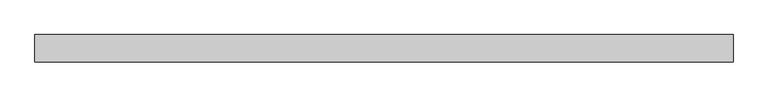
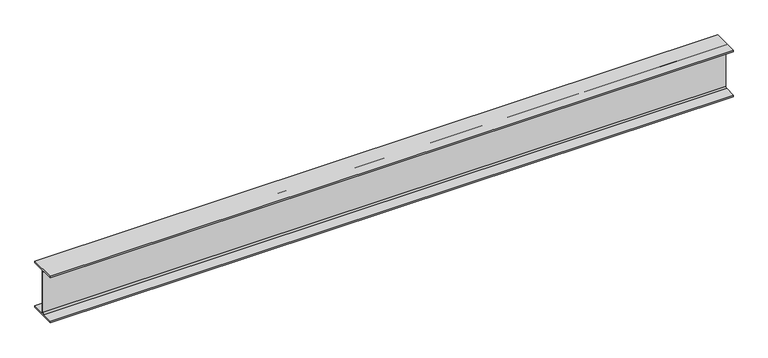
"""IFC4 building model written with IfcOpenShell, lengths in millimetres: beam geometry, Old_Steel Beam_H-KSD3502 : H_SB_ASB_H-482×300x11x15."""

import ifcopenshell
import ifcopenshell.guid

model = None  # the IFC model being written
_history = None  # IfcOwnerHistory: only IFC2X3 demands one
_inside = {}  # id of a spatial element -> (the spatial element, [elements in it])
_under = {}  # id of a project, library or spatial element -> (it, [spatial elements below it])
_declared = {}  # id of a project -> (the project, [libraries it declares])
_typed = {}  # id of a type object -> (the type object, [elements of that type])
_made_of = {}  # id of a material, layer set ... -> (it, [elements and type objects made of it])


def new_model(schema):
    """Start an empty IFC model of exactly this schema.

    Asked for "IFC4X3", IfcOpenShell would pick the latest addendum, in which some entities
    have other attributes; the version numbers below select the first issue.
    IFC2X3 requires an IfcOwnerHistory on every rooted entity: one is made here for all.
    """
    global model, _history
    if schema == "IFC4X3":
        model = ifcopenshell.file(schema_version=(4, 3, 0, 0))
    else:
        model = ifcopenshell.file(schema=schema)
    _inside.clear()
    _under.clear()
    _declared.clear()
    _typed.clear()
    _made_of.clear()
    _history = None
    if model.schema == "IFC2X3":
        org = make("IfcOrganization", Name="unknown")
        user = make(
            "IfcPersonAndOrganization",
            ThePerson=make("IfcPerson", FamilyName="unknown"),
            TheOrganization=org,
        )
        app = make(
            "IfcApplication",
            ApplicationDeveloper=org,
            Version="unknown",
            ApplicationFullName="unknown",
            ApplicationIdentifier="unknown",
        )
        _history = make(
            "IfcOwnerHistory",
            OwningUser=user,
            OwningApplication=app,
            ChangeAction="ADDED",
            CreationDate=0,
        )
    return model


def make(cls, **values):
    """One entity of the class cls with the attributes given. An attribute that is None is left unset."""
    return model.create_entity(
        cls, **{name: value for name, value in values.items() if value is not None}
    )


def rooted(cls, **values):
    """An entity with a GlobalId (a new one), such as an element, a storey or a relation."""
    return make(cls, GlobalId=ifcopenshell.guid.new(), OwnerHistory=_history, **values)


def si_unit(unit_type, name, prefix=None):
    """IfcSIUnit, for example si_unit("LENGTHUNIT", "METRE", prefix="MILLI")."""
    return make("IfcSIUnit", UnitType=unit_type, Prefix=prefix, Name=name)


def assignment(units):
    """IfcUnitAssignment: the units of a project."""
    return None if units is None else make("IfcUnitAssignment", Units=units)


def point(xyz):
    """IfcCartesianPoint."""
    return None if xyz is None else make("IfcCartesianPoint", Coordinates=xyz)


def direction(xyz):
    """IfcDirection."""
    return None if xyz is None else make("IfcDirection", DirectionRatios=xyz)


def frame(location, z_axis=None, x_axis=None):
    """IfcAxis2Placement3D, a coordinate frame: its origin and axes. An axis left out is left unset."""
    return make(
        "IfcAxis2Placement3D",
        Location=point(location),
        Axis=direction(z_axis),
        RefDirection=direction(x_axis),
    )


def frame_2d(location, x_axis=None):
    """IfcAxis2Placement2D, a coordinate frame in the plane: its origin and x axis."""
    return make(
        "IfcAxis2Placement2D", Location=point(location), RefDirection=direction(x_axis)
    )


def origin():
    """The frame at (0, 0, 0) with its axes left unset."""
    return frame((0.0, 0.0, 0.0))


def place(relative_to, where):
    """IfcLocalPlacement: puts the frame where relative to a parent placement (None: the world)."""
    return make(
        "IfcLocalPlacement", PlacementRelTo=relative_to, RelativePlacement=where
    )


def context(
    kind, dimensions, precision=None, world=None, true_north=None, identifier=None
):
    """IfcGeometricRepresentationContext, for example the 3D "Model" context."""
    return make(
        "IfcGeometricRepresentationContext",
        ContextIdentifier=identifier,
        ContextType=kind,
        CoordinateSpaceDimension=dimensions,
        Precision=precision,
        WorldCoordinateSystem=world,
        TrueNorth=true_north,
    )


def project(units=None, contexts=None):
    """IfcProject with its units and contexts."""
    return rooted(
        "IfcProject",
        Name="project",
        RepresentationContexts=contexts,
        UnitsInContext=assignment(units),
    )


def spatial(cls, under=None, at=None, **own):
    """A site, building, storey or space (cls), placed at a placement, below another one or the project."""
    s = rooted(cls, ObjectPlacement=at, **own)
    if under is not None:
        _under.setdefault(under.id(), (under, []))[1].append(s)
    return s


def polyline(points):
    """IfcPolyline through the points."""
    return make("IfcPolyline", Points=[point(p) for p in points])


def circle_curve(where, radius):
    """IfcCircle in the frame where."""
    return make("IfcCircle", Position=where, Radius=radius)


def trimmed(basis, trim1, trim2, sense, master):
    """IfcTrimmedCurve: the piece of a basis curve between two trims."""
    return make(
        "IfcTrimmedCurve",
        BasisCurve=basis,
        Trim1=trim1,
        Trim2=trim2,
        SenseAgreement=sense,
        MasterRepresentation=master,
    )


def segment(curve, same_sense, transition):
    """IfcCompositeCurveSegment."""
    return make(
        "IfcCompositeCurveSegment",
        Transition=transition,
        SameSense=same_sense,
        ParentCurve=curve,
    )


def composite_curve(segments, self_intersect=None):
    """IfcCompositeCurve: segments joined end to end."""
    return make("IfcCompositeCurve", Segments=segments, SelfIntersect=self_intersect)


def outline(outer, holes=None, kind="AREA"):
    """IfcArbitraryClosedProfileDef: a profile drawn as a closed curve; with holes, ...WithVoids."""
    if holes is None:
        return make("IfcArbitraryClosedProfileDef", ProfileType=kind, OuterCurve=outer)
    return make(
        "IfcArbitraryProfileDefWithVoids",
        ProfileType=kind,
        OuterCurve=outer,
        InnerCurves=holes,
    )


def extrude(swept, where, along, depth):
    """IfcExtrudedAreaSolid: the profile swept, set in the frame where, extruded along a direction by depth."""
    return make(
        "IfcExtrudedAreaSolid",
        SweptArea=swept,
        Position=where,
        ExtrudedDirection=direction(along),
        Depth=depth,
    )


def shape(context_of_items, identifier, shape_type, items):
    """IfcShapeRepresentation: the items that make up one representation, for example the "Body"."""
    return make(
        "IfcShapeRepresentation",
        ContextOfItems=context_of_items,
        RepresentationIdentifier=identifier,
        RepresentationType=shape_type,
        Items=items,
    )


def source(mapping_origin, context_of_items, identifier, shape_type, items):
    """IfcRepresentationMap: a shape defined once, which mapped items show again and again."""
    return make(
        "IfcRepresentationMap",
        MappingOrigin=mapping_origin,
        MappedRepresentation=shape(context_of_items, identifier, shape_type, items),
    )


def transform(
    local_origin,
    x_axis=None,
    y_axis=None,
    z_axis=None,
    scale=None,
    scale2=None,
    scale3=None,
    uniform=True,
):
    """IfcCartesianTransformationOperator3D, or its non-uniform kind. x_axis, y_axis, z_axis: its Axis1, 2, 3."""
    if uniform:
        return make(
            "IfcCartesianTransformationOperator3D",
            Axis1=direction(x_axis),
            Axis2=direction(y_axis),
            LocalOrigin=point(local_origin),
            Scale=scale,
            Axis3=direction(z_axis),
        )
    return make(
        "IfcCartesianTransformationOperator3DnonUniform",
        Axis1=direction(x_axis),
        Axis2=direction(y_axis),
        LocalOrigin=point(local_origin),
        Scale=scale,
        Axis3=direction(z_axis),
        Scale2=scale2,
        Scale3=scale3,
    )


def mapped(mapping_source, mapping_target):
    """IfcMappedItem: shows the shape of a source again, moved by a transform."""
    return make(
        "IfcMappedItem", MappingSource=mapping_source, MappingTarget=mapping_target
    )


def made_of(thing, what):
    """Note that an element or type object is made of a material, layer set ...; save() writes the relation."""
    if what is not None:
        _made_of.setdefault(what.id(), (what, []))[1].append(thing)
    return thing


def element(
    cls,
    number,
    at=None,
    inside=None,
    cuts=None,
    type_object=None,
    material=None,
    context=None,
    identifier="Body",
    shape_type=None,
    held_by="IfcProductDefinitionShape",
    body=None,
    shapes=None,
    **own,
):
    """One element of the class cls, such as IfcWall. Its Tag is "e" and its number.

    at: its placement. inside: the storey or other place that contains it. cuts: it is an
    opening in that element (IfcRelVoidsElement). A single representation is given by context,
    identifier, shape_type and body (its items); several are given by shapes. held_by: the class
    of the entity that holds the representations. save() writes the other relations.
    """
    e = rooted(cls, Tag="e%d" % number, ObjectPlacement=at, **own)
    if body is not None:
        shapes = [shape(context, identifier, shape_type, body)]
    if shapes is not None:
        e.Representation = make(held_by, Representations=shapes)
    if inside is not None:
        _inside.setdefault(inside.id(), (inside, []))[1].append(e)
    if cuts is not None:
        rooted(
            "IfcRelVoidsElement", RelatingBuildingElement=cuts, RelatedOpeningElement=e
        )
    if type_object is not None:
        _typed.setdefault(type_object.id(), (type_object, []))[1].append(e)
    return made_of(e, material)


def aggregate(whole, parts):
    """IfcRelAggregates: a whole, such as a stair, and the parts it consists of."""
    return rooted("IfcRelAggregates", RelatingObject=whole, RelatedObjects=parts)


def save(model, path):
    """Write the relations noted so far, then the file.

    IfcRelAggregates (storeys below a building ...), IfcRelContainedInSpatialStructure (elements
    in a storey), IfcRelDefinesByType, IfcRelAssociatesMaterial and IfcRelDeclares: one each for
    every whole, place, type object, material and project.
    """
    for whole, parts in _under.values():
        aggregate(whole, parts)
    for where, things in _inside.values():
        rooted(
            "IfcRelContainedInSpatialStructure",
            RelatedElements=things,
            RelatingStructure=where,
        )
    for kind, things in _typed.values():
        rooted("IfcRelDefinesByType", RelatedObjects=things, RelatingType=kind)
    for what, things in _made_of.values():
        rooted("IfcRelAssociatesMaterial", RelatedObjects=things, RelatingMaterial=what)
    for by, libraries in _declared.values():
        rooted("IfcRelDeclares", RelatingContext=by, RelatedDefinitions=libraries)
    model.write(path)


def beam_e084cd09(model_context):
    return source(origin(), model_context, "Body", "SweptSolid", [
        extrude(outline(composite_curve([segment(polyline([(82.5, -141.5), (82.5, -151.7), (-82.5, -151.7), (-82.5, -141.5), (-11.9, -141.5)]), True, "CONTINUOUS"), segment(trimmed(circle_curve(frame_2d((-11.9, -132.6)), 8.9), [point((-11.9, -141.5))], [point((-3.0, -132.6))], True, "CARTESIAN"), True, "CONTINUOUS"), segment(polyline([(-3.0, -132.6), (-3.0, 132.6)]), True, "CONTINUOUS"), segment(trimmed(circle_curve(frame_2d((-11.9, 132.6)), 8.9), [point((-3.0, 132.6))], [point((-11.9, 141.5))], True, "CARTESIAN"), True, "CONTINUOUS"), segment(polyline([(-11.9, 141.5), (-82.5, 141.5), (-82.5, 151.7), (82.5, 151.7), (82.5, 141.5), (11.9, 141.5)]), True, "CONTINUOUS"), segment(trimmed(circle_curve(frame_2d((11.9, 132.6)), 8.9), [point((11.9, 141.5))], [point((3.0, 132.6))], True, "CARTESIAN"), True, "CONTINUOUS"), segment(polyline([(3.0, 132.6), (3.0, -132.6)]), True, "CONTINUOUS"), segment(trimmed(circle_curve(frame_2d((11.9, -132.6)), 8.9), [point((3.0, -132.6))], [point((11.9, -141.5))], True, "CARTESIAN"), True, "CONTINUOUS"), segment(polyline([(11.9, -141.5), (82.5, -141.5)]), True, "CONTINUOUS")], self_intersect=False)), frame((-2212.3, 0.0, 0.0), z_axis=(1.0, 0.0, 0.0), x_axis=(0.0, 1.0, 0.0)), (0.0, 0.0, 1.0), 4224.6),
    ])


if __name__ == "__main__":
    model = new_model("IFC4")
    model_context = context("Model", 3, world=origin())
    ifc_project = project(units=[si_unit("LENGTHUNIT", "METRE", prefix="MILLI")], contexts=[model_context])
    site = spatial("IfcSite", under=ifc_project)
    building = spatial("IfcBuilding", under=site)
    placement = place(None, origin())
    beam_shape = beam_e084cd09(model_context)
    element("IfcBeam", 1, ObjectType="Old_Steel Beam_H-KSD3502 : H_SB_ASB_H-482×300x11x15", at=placement, inside=building, context=model_context, shape_type="MappedRepresentation", body=[
        mapped(beam_shape, transform((0.0, 0.0, 0.0), x_axis=(1.0, 0.0, 0.0), y_axis=(0.0, 1.0, 0.0), z_axis=(0.0, 0.0, 1.0))),
    ])
    save(model, "model.ifc")

# Revit data of these elements
# Type "Old_Steel Beam_H-KSD3502 : H_SB_ASB_H-482×300x11x15"
#   Width = 30.0 cm
#   Web Thickness = 1.1 cm
#   Web Fillet = 2.6 cm
#   Warping Constant = 3680250.0 cm⁶
#   Torsional Moment of Inertia = 88.2192 cm⁴
#   Torsional Modulus = 1.0 cm³
#   Section Area = 145.5 cm²
#   Plastic Modulus weak axis = 695.0 cm³
#   Plastic Modulus strong axis = 2790.0 cm³
#   Perimeter = 2.10 m²/m
#   Nominal Weight = 114.00 kgf/m
#   Moment of Inertia weak axis = 6760.00 cm⁴
#   Moment of Inertia strong axis = 60400.00 cm⁴
#   Height = 48.2 cm
#   Flange Thickness = 1.5 cm
#   Elastic Modulus weak axis = 451.0 cm³
#   Elastic Modulus strong axis = 2500.0 cm³
#   Centroid Vertical = 24.1 cm
#   Centroid Horizontal = 15.0 cm
#   Length [instance default] = 1.5240 m
#   Structural Material [instance default] = Steel, 45-345
#   Assembly Code = ""
# Element 1 (IfcBeam, "Old_Steel Beam_H-KSD3502 : H_SB_ASB_H-482×300x11x15")
#   Structural Material = none
# Materials
#   "Steel, 45-345": class "Metal", colour RGB 189 187 185, transparency 0, Description = "Steel 345 MPa", Cost = 0
